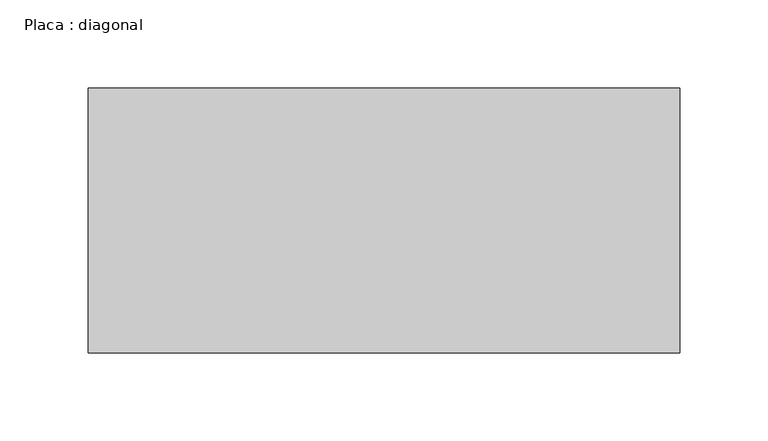
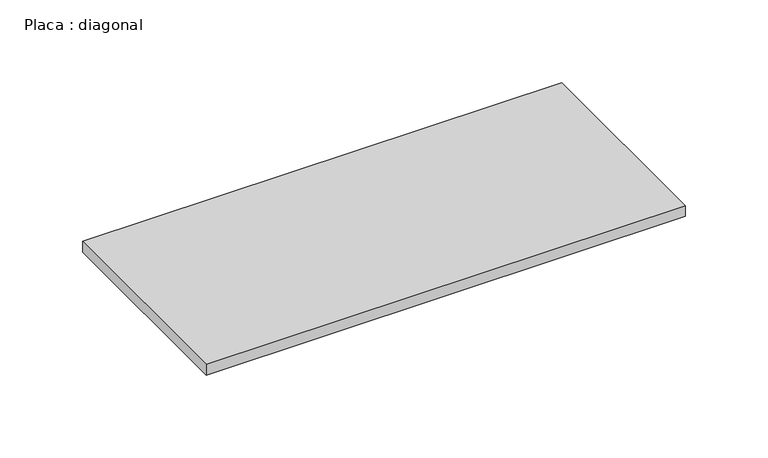
"""IFC4 building model written with IfcOpenShell, lengths in millimetres: beam geometry, Placa : diagonal."""

from ifc_helpers import new_model, si_unit, frame, origin, place, context, project, spatial, polyline, outline, extrude, source, transform, mapped, element, save


def placa_diagonal_41f6052a(model_context):
    return source(origin(), model_context, "Body", "SweptSolid", [
        extrude(outline(polyline([(167.3896443, 75.0), (167.3896443, -75.0), (-167.5872499, -75.0), (-167.5872499, 75.0), (167.3896443, 75.0)])), frame((0.0, 0.0, -4.0), z_axis=(0.0, 0.0, 1.0), x_axis=(1.0, 0.0, 0.0)), (0.0, 0.0, 1.0), 8.0),
    ])


if __name__ == "__main__":
    model = new_model("IFC4")
    model_context = context("Model", 3, world=origin())
    ifc_project = project(units=[si_unit("LENGTHUNIT", "METRE", prefix="MILLI")], contexts=[model_context])
    site = spatial("IfcSite", under=ifc_project)
    building = spatial("IfcBuilding", under=site)
    placement = place(None, origin())
    placa_diagonal_shape = placa_diagonal_41f6052a(model_context)
    element("IfcBeam", 1, ObjectType="Placa : diagonal", at=placement, inside=building, context=model_context, shape_type="MappedRepresentation", body=[
        mapped(placa_diagonal_shape, transform((0.0, 0.0, 0.0), x_axis=(1.0, 0.0, 0.0), y_axis=(0.0, 1.0, 0.0), z_axis=(0.0, 0.0, 1.0))),
    ])
    save(model, "model.ifc")

# Revit data of these elements
# Type "Placa : diagonal"
#   W = 0
#   Length [instance default] = 1.50 m
#   b = 0.15 m
#   d = 0.008 m
#   A = 0 m²
#   Structural Material [instance default] = Aço, 45-345
# Element 1 (IfcBeam, "Placa : diagonal")
#   Materials on its faces: "Aço, 45-345"
# Materials
#   "Aço, 45-345": class "Metal", colour RGB 247 247 247, transparency 0, Description = "Aço 345 MPa", Cost = 0
